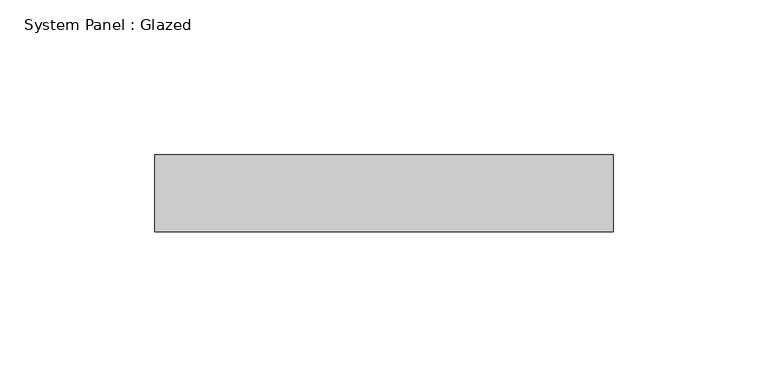
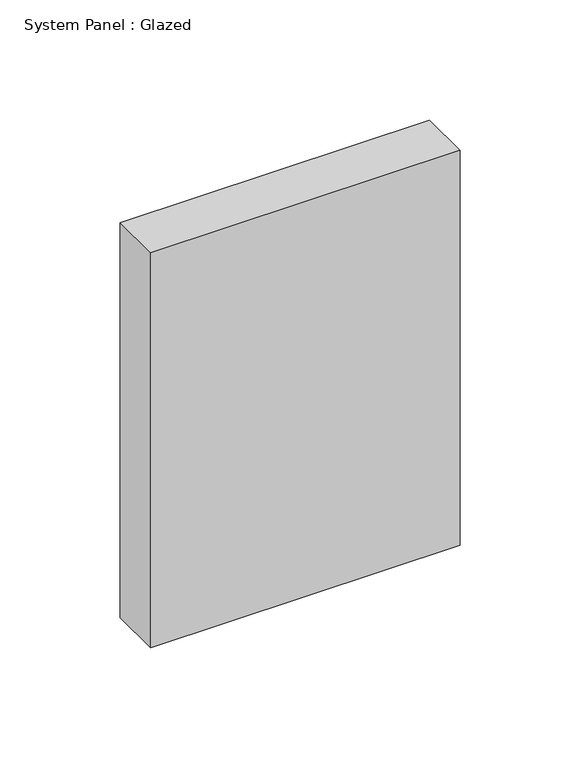
"""IFC4 building model written with IfcOpenShell, lengths in millimetres: plate geometry, System Panel : Glazed."""

from ifc_helpers import new_model, si_unit, origin, origin_with_axes, place, context, project, spatial, polyline, outline, extrude, source, transform, mapped, element, save


def system_panel_glazed_2ba9a9ff(model_context):
    return source(origin(), model_context, "Body", "SweptSolid", [
        extrude(outline(polyline([(74.1536727, 24.5), (-74.1536727, 24.5), (-74.1536727, 49.5), (74.1536727, 49.5), (74.1536727, 24.5)])), origin_with_axes(), (0.0, 0.0, 1.0), 200.0),
    ])


if __name__ == "__main__":
    model = new_model("IFC4")
    model_context = context("Model", 3, world=origin())
    ifc_project = project(units=[si_unit("LENGTHUNIT", "METRE", prefix="MILLI")], contexts=[model_context])
    site = spatial("IfcSite", under=ifc_project)
    building = spatial("IfcBuilding", under=site)
    placement = place(None, origin())
    system_panel_glazed_shape = system_panel_glazed_2ba9a9ff(model_context)
    element("IfcPlate", 1, ObjectType="System Panel : Glazed", at=placement, inside=building, context=model_context, shape_type="MappedRepresentation", body=[
        mapped(system_panel_glazed_shape, transform((0.0, 0.0, 0.0), x_axis=(1.0, 0.0, 0.0), y_axis=(0.0, 1.0, 0.0), z_axis=(0.0, 0.0, 1.0))),
    ])
    save(model, "model.ifc")

# Revit data of these elements
# Element 1 (IfcPlate, "System Panel : Glazed")
#   Materials on its faces: "Glass"
# Materials
#   "Glass": class "Glass", colour RGB 218 227 224, transparency 0.85, Description = "Soda Lime Glass", Cost = 0
